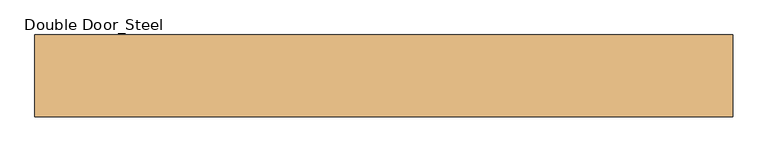
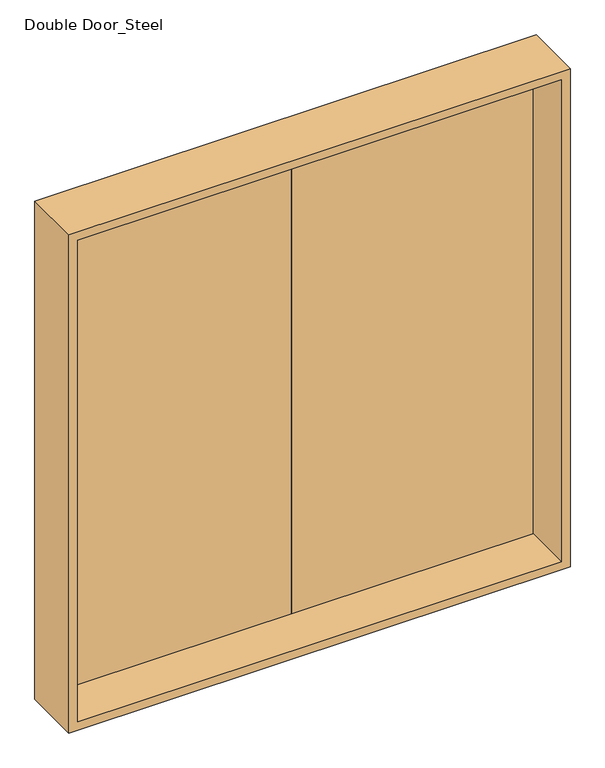
"""IFC4 building model written with IfcOpenShell, lengths in millimetres: door geometry, Double Door_Steel : H_DR_AMB_Double Door_Steel_W2000xH2100."""

from ifc_helpers import new_model, si_unit, frame, origin, place, context, project, spatial, polyline, outline, extrude, faceted_brep, source, transform, mapped, element, save


def double_door_steel_cbf312ec(model_context):
    return source(origin(), model_context, "Body", "SolidModel", [
        extrude(outline(polyline([(980.0, 77.0), (0.0, 77.0), (0.0, 117.0), (980.0, 117.0), (980.0, 77.0)])), frame((0.0, 0.0, 20.0), z_axis=(0.0, 0.0, 1.0), x_axis=(1.0, 0.0, 0.0)), (0.0, 0.0, 1.0), 2060.0),
        extrude(outline(polyline([(0.0, 77.0), (-980.0, 77.0), (-980.0, 117.0), (0.0, 117.0), (0.0, 77.0)])), frame((0.0, 0.0, 20.0), z_axis=(0.0, 0.0, 1.0), x_axis=(1.0, 0.0, 0.0)), (0.0, 0.0, 1.0), 2060.0),
        faceted_brep([(1000.0, -117.0, 2100.0), (1000.0, 117.0, 2100.0), (-1000.0, 117.0, 2100.0), (-1000.0, -117.0, 2100.0), (965.0, 77.0, 2065.0), (965.0, -117.0, 2065.0), (-965.0, -117.0, 2065.0), (-965.0, 77.0, 2065.0), (980.0, 117.0, 2080.0), (980.0, 77.0, 2080.0), (-980.0, 77.0, 2080.0), (-980.0, 117.0, 2080.0), (-1000.0, 117.0, 0.0), (-1000.0, -117.0, 0.0), (-965.0, -117.0, 35.0), (-965.0, 77.0, 35.0), (-980.0, 77.0, 20.0), (-980.0, 117.0, 20.0), (1000.0, 117.0, 0.0), (980.0, 117.0, 20.0), (1000.0, -117.0, 0.0), (965.0, -117.0, 35.0), (965.0, 77.0, 35.0), (980.0, 77.0, 20.0)], [[[0, 1, 2, 3]], [[4, 5, 6, 7]], [[8, 9, 10, 11]], [[3, 2, 12, 13]], [[7, 6, 14, 15]], [[11, 10, 16, 17]], [[18, 12, 2, 1], [8, 11, 17, 19]], [[13, 12, 18, 20]], [[0, 3, 13, 20], [21, 14, 6, 5]], [[15, 14, 21, 22]], [[23, 16, 10, 9], [4, 7, 15, 22]], [[17, 16, 23, 19]], [[20, 18, 1, 0]], [[22, 21, 5, 4]], [[19, 23, 9, 8]]]),
    ])


if __name__ == "__main__":
    model = new_model("IFC4")
    model_context = context("Model", 3, world=origin())
    ifc_project = project(units=[si_unit("LENGTHUNIT", "METRE", prefix="MILLI")], contexts=[model_context])
    site = spatial("IfcSite", under=ifc_project)
    building = spatial("IfcBuilding", under=site)
    placement = place(None, origin())
    double_door_steel_shape = double_door_steel_cbf312ec(model_context)
    element("IfcDoor", 1, ObjectType="Double Door_Steel : H_DR_AMB_Double Door_Steel_W2000xH2100", at=placement, inside=building, context=model_context, shape_type="MappedRepresentation", body=[
        mapped(double_door_steel_shape, transform((0.0, 0.0, 0.0), x_axis=(1.0, 0.0, 0.0), y_axis=(0.0, 1.0, 0.0), z_axis=(0.0, 0.0, 1.0))),
    ])
    save(model, "model.ifc")

# Revit data of these elements
# Type "Double Door_Steel : H_DR_AMB_Double Door_Steel_W2000xH2100"
#   Type Mark = ""
#   프레임 = ""
#   철물 = ""
#   유리/마감 = ""
#   위치/개소 = ""
#   부호 = "1/SD"
#   문번호 = ""
#   문기호 = "SD"
#   Analytic Construction = "<None>"
#   Height = 2100.000 mm
#   Width = 2000.000 mm
#   Define Thermal Properties by = 1
#   문 틀 = none
#   문 = none
#   Function = (empty or 0)
#   Assembly Code = ""
#   Wall Closure = (empty or 0)
